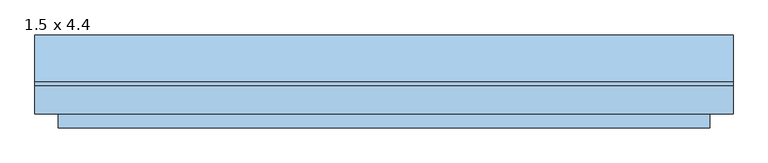
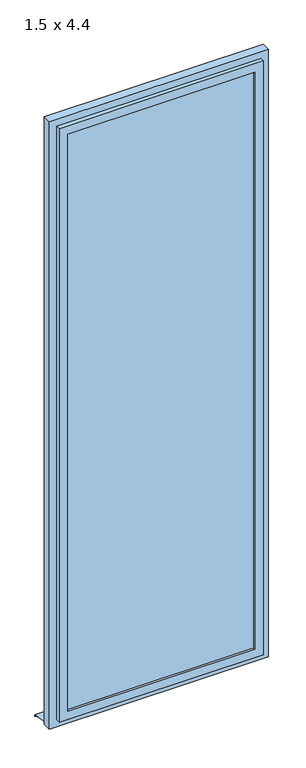
"""IFC4 building model written with IfcOpenShell, lengths in millimetres: window geometry, Fenstertür 1-flg : 1.5 x 4.4."""

from ifc_helpers import new_model, si_unit, frame, origin, place, context, project, spatial, polyline, outline, extrude, faceted_brep, source, transform, mapped, element, save


def window_1_5_x_4_4_ca739f39(model_context):
    return source(origin(), model_context, "Body", "SolidModel", [
        extrude(outline(polyline([(4400.0, 750.0), (4400.0, -750.0), (0.0, -750.0), (0.0, 750.0), (4400.0, 750.0)]), holes=[polyline([(4320.0, 670.0), (80.0, 670.0), (80.0, -670.0), (4320.0, -670.0), (4320.0, 670.0)])]), frame((0.0, 60.0, 0.0), z_axis=(0.0, 1.0, 0.0), x_axis=(0.0, 0.0, 1.0)), (0.0, 0.0, 1.0), 60.0),
        faceted_brep([(700.0, 60.0, 4350.0), (700.0, 30.0, 4350.0), (700.0, 30.0, 50.0), (700.0, 60.0, 50.0), (-700.0, 30.0, 4350.0), (-700.0, 30.0, 50.0), (640.0, 30.0, 110.0), (-640.0, 30.0, 110.0), (-640.0, 30.0, 4290.0), (640.0, 30.0, 4290.0), (-700.0, 60.0, 50.0), (-700.0, 60.0, 4350.0), (670.0, 60.0, 4320.0), (-670.0, 60.0, 4320.0), (-670.0, 60.0, 80.0), (670.0, 60.0, 80.0), (670.0, 90.0, 4320.0), (670.0, 90.0, 80.0), (-670.0, 90.0, 80.0), (-670.0, 90.0, 4320.0), (640.0, 90.0, 4290.0), (-640.0, 90.0, 4290.0), (-640.0, 90.0, 110.0), (640.0, 90.0, 110.0)], [[[0, 1, 2, 3]], [[1, 4, 5, 2], [6, 7, 8, 9]], [[3, 2, 5, 10]], [[3, 10, 11, 0], [12, 13, 14, 15]], [[16, 12, 15, 17]], [[17, 15, 14, 18]], [[17, 18, 19, 16], [20, 21, 22, 23]], [[9, 20, 23, 6]], [[6, 23, 22, 7]], [[10, 5, 4, 11]], [[18, 14, 13, 19]], [[7, 22, 21, 8]], [[11, 4, 1, 0]], [[19, 13, 12, 16]], [[8, 21, 20, 9]]]),
        extrude(outline(polyline([(130.0221543, 20.0), (230.0, 0.0), (230.0, -10.0), (228.0, -10.0), (228.0, -1.6395366), (129.8240723, 18.0), (120.0, 18.0), (120.0, 20.0), (130.0221543, 20.0)])), frame((-750.0, 0.0, 0.0), z_axis=(1.0, 0.0, 0.0), x_axis=(0.0, 1.0, 0.0)), (0.0, 0.0, 1.0), 1500.0),
        extrude(outline(polyline([(640.0, 45.0), (-640.0, 45.0), (-640.0, 75.0), (640.0, 75.0), (640.0, 45.0)])), frame((0.0, 0.0, 110.0), z_axis=(0.0, 0.0, 1.0), x_axis=(1.0, 0.0, 0.0)), (0.0, 0.0, 1.0), 4180.0),
    ])


if __name__ == "__main__":
    model = new_model("IFC4")
    model_context = context("Model", 3, world=origin())
    ifc_project = project(units=[si_unit("LENGTHUNIT", "METRE", prefix="MILLI")], contexts=[model_context])
    site = spatial("IfcSite", under=ifc_project)
    building = spatial("IfcBuilding", under=site)
    placement = place(None, origin())
    window_1_5_x_4_4_shape = window_1_5_x_4_4_ca739f39(model_context)
    element("IfcWindow", 1, ObjectType="Fenstertür 1-flg : 1.5 x 4.4", at=placement, inside=building, context=model_context, shape_type="MappedRepresentation", body=[
        mapped(window_1_5_x_4_4_shape, transform((0.0, 0.0, 0.0), x_axis=(1.0, 0.0, 0.0), y_axis=(0.0, 1.0, 0.0), z_axis=(0.0, 0.0, 1.0))),
    ])
    save(model, "model.ifc")

# Revit data of these elements
# Type "Fenstertür 1-flg : 1.5 x 4.4"
#   Type Mark = "58"
#   Operation = "SinglePanel"
#   Construction Type Id = "GSP4R"
#   Keynote = "16.05.01"
#   Analytic Construction = "1/8 Zoll Pilkington-Verglasung einfach"
#   Visual Light Transmittance = 0.9
#   Thermal Resistance (R) = 0.1491 (m²·K)/W
#   Solar Heat Gain Coefficient = 0.86
#   Rough Width = 1.500 m
#   Rough Height = 4.400 m
#   Heat Transfer Coefficient (U) = 6.7069 W/(m²·K)
#   Rahmentiefe = 0.060 m
#   Rahmenhöhe - unten = 0.080 m
#   Rahmenhöhe - oben = 0.080 m
#   Rahmenbreite = 0.080 m
#   Height = 4.400 m
#   Tiefe Flügel = 0.060 m
#   Flügelbreite = 0.060 m
#   Einbautiefe (von außen) [instance default] = 0.080 m
#   Width = 1.500 m
#   Kippflügel [instance default] = yes
#   Drehflügel im Grundriss darstellen [instance default] = yes
#   Drehflügel 1 [instance default] = yes
#   Rahmen 1 [instance default] = none
#   Glas [instance default] = none
#   Flügel [instance default] = none
#   Fensterbank Außenseite [instance default] = none
#   Wall Closure = (empty or 0)
# Element 1 (IfcWindow, "Fenstertür 1-flg : 1.5 x 4.4")
#   Materials on its faces: "Kunststoff - Weiß", "Glas"
# Materials
#   "Kunststoff - Weiß": class "Kunststoff", colour RGB 249 249 249, transparency 0, Cost = 0
#   "Glas": class "Glas", colour RGB 0 0 255, transparency 0.75, Comments = "Render-Darstellung nicht aktualisiert ", Cost = 0
